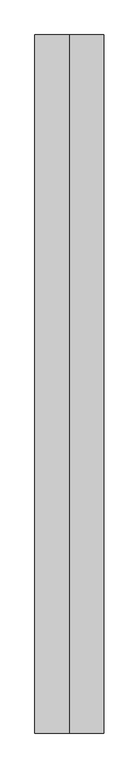
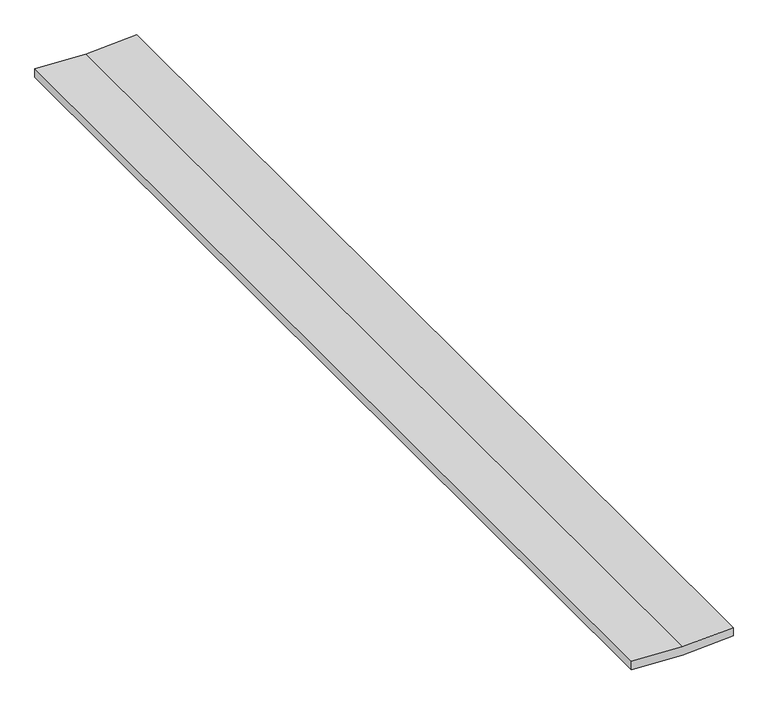
"""IFC4 building model written with IfcOpenShell, lengths in millimetres: proxy geometry, COVER BOARD001 3887 : COVER BOARD001 3887."""

from ifc_helpers import new_model, si_unit, frame, origin, place, context, project, spatial, polyline, outline, extrude, source, transform, mapped, element, save


def generic_models_2390c736(model_context):
    return source(origin(), model_context, "Body", "SweptSolid", [
        extrude(outline(polyline([(40228.3444286, -4699.8063764), (40233.346, -4797.9038825), (40216.0142809, -4797.9038825), (40211.0127094, -4699.8063764), (40216.0142809, -4601.0538825), (40233.346, -4601.0538825), (40228.3444286, -4699.8063764)])), frame((0.0, -1052.6406573, 0.0), z_axis=(0.0, 1.0, 0.0), x_axis=(0.0, 0.0, 1.0)), (0.0, 0.0, 1.0), 2000.0),
    ])


if __name__ == "__main__":
    model = new_model("IFC4")
    model_context = context("Model", 3, world=origin())
    ifc_project = project(units=[si_unit("LENGTHUNIT", "METRE", prefix="MILLI")], contexts=[model_context])
    site = spatial("IfcSite", under=ifc_project)
    building = spatial("IfcBuilding", under=site)
    placement = place(None, origin())
    generic_models_shape = generic_models_2390c736(model_context)
    element("IfcBuildingElementProxy", 1, Name="COVER BOARD001 3887 : COVER BOARD001 3887", ObjectType="COVER BOARD001 3887 : COVER BOARD001 3887", at=placement, inside=building, context=model_context, shape_type="MappedRepresentation", body=[
        mapped(generic_models_shape, transform((0.0, 0.0, 0.0), x_axis=(1.0, 0.0, 0.0), y_axis=(0.0, 1.0, 0.0), z_axis=(0.0, 0.0, 1.0))),
    ])
    save(model, "model.ifc")

# Revit data of these elements
# Type "COVER BOARD001 3887 : COVER BOARD001 3887"
#   NameOverride = "COVER BOARD001"
# Element 1 (IfcBuildingElementProxy, "COVER BOARD001 3887 : COVER BOARD001 3887")
#   Materials on its faces: "CDX PLYWOOD - SEE STRUCTURAL DWGS"
# Materials
#   "CDX PLYWOOD - SEE STRUCTURAL DWGS": class "Unassigned", colour RGB 138 93 50, transparency 0, Cost = 0
